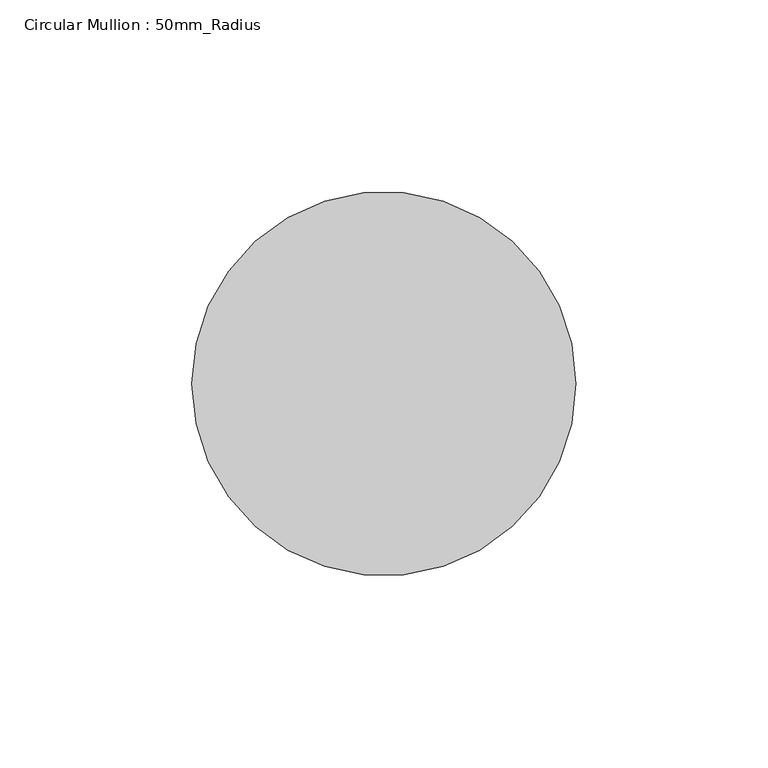
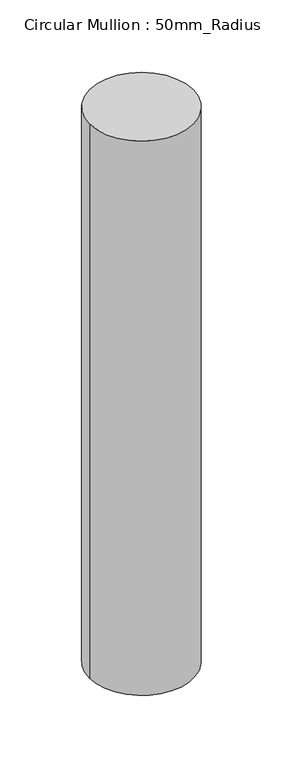
"""IFC4 building model written with IfcOpenShell, lengths in millimetres: member geometry, Circular Mullion : 50mm_Radius."""

from ifc_helpers import new_model, si_unit, point, frame, origin, origin_2d, place, context, project, spatial, circle_curve, trimmed, segment, composite_curve, outline, extrude, source, transform, mapped, element, save


def circular_mullion_50mm_radius_b33f9675(model_context):
    return source(origin(), model_context, "Body", "SweptSolid", [
        extrude(outline(composite_curve([segment(trimmed(circle_curve(origin_2d(), 50.0), [point((50.0, 0.0))], [point((-50.0, 0.0))], False, "CARTESIAN"), True, "CONTINUOUS"), segment(trimmed(circle_curve(origin_2d(), 50.0), [point((-50.0, 0.0))], [point((50.0, 0.0))], False, "CARTESIAN"), True, "CONTINUOUS")], self_intersect=False)), frame((0.0, 0.0, -564.9999997), z_axis=(0.0, 0.0, 1.0), x_axis=(1.0, 0.0, 0.0)), (0.0, 0.0, 1.0), 564.9999997),
    ])


if __name__ == "__main__":
    model = new_model("IFC4")
    model_context = context("Model", 3, world=origin())
    ifc_project = project(units=[si_unit("LENGTHUNIT", "METRE", prefix="MILLI")], contexts=[model_context])
    site = spatial("IfcSite", under=ifc_project)
    building = spatial("IfcBuilding", under=site)
    placement = place(None, origin())
    circular_mullion_50mm_radius_shape = circular_mullion_50mm_radius_b33f9675(model_context)
    element("IfcMember", 1, ObjectType="Circular Mullion : 50mm_Radius", at=placement, inside=building, context=model_context, shape_type="MappedRepresentation", body=[
        mapped(circular_mullion_50mm_radius_shape, transform((0.0, 0.0, 0.0), x_axis=(1.0, 0.0, 0.0), y_axis=(0.0, 1.0, 0.0), z_axis=(0.0, 0.0, 1.0))),
    ])
    save(model, "model.ifc")

# Revit data of these elements
# Type "Circular Mullion : 50mm_Radius"
#   Keynote = "H11"
#   built-in parameter 1007350 = 0.164042 (stored number, unit not read)
# Element 1 (IfcMember, "Circular Mullion : 50mm_Radius")
#   Materials on its faces: "Aluminium"
# Materials
#   "Aluminium": class "Metal", colour RGB 247 247 247, transparency 0, Description = "Aluminium 6061", Cost = 0
